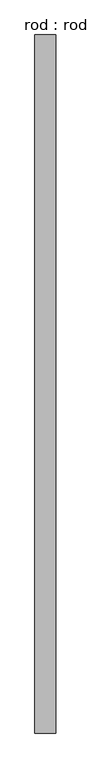
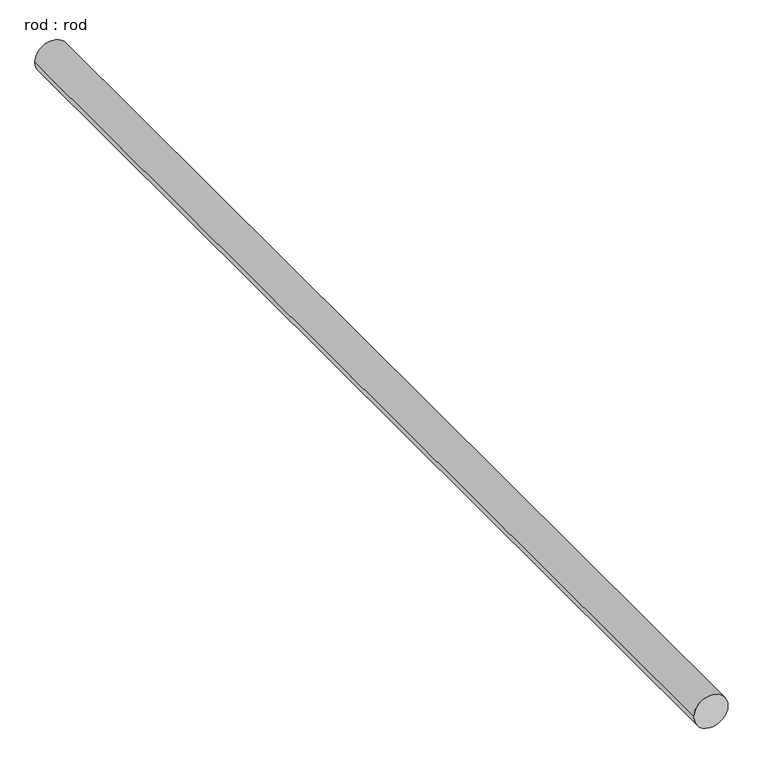
"""IFC4 building model written with IfcOpenShell, lengths in millimetres: proxy geometry, rod : rod."""

from ifc_helpers import new_model, si_unit, point, frame, frame_2d, origin, place, context, project, spatial, circle_curve, trimmed, segment, composite_curve, outline, extrude, source, transform, mapped, element, save


def rod_rod_c0b6d43a(model_context):
    return source(origin(), model_context, "Body", "SweptSolid", [
        extrude(outline(composite_curve([segment(trimmed(circle_curve(frame_2d((0.0108462, 0.0)), 200.0), [point((0.0108462, 200.0))], [point((0.0108462, -200.0))], False, "CARTESIAN"), True, "CONTINUOUS"), segment(trimmed(circle_curve(frame_2d((0.0108462, 0.0)), 200.0), [point((0.0108462, -200.0))], [point((0.0108462, 200.0))], False, "CARTESIAN"), True, "CONTINUOUS")], self_intersect=False)), frame((0.0, -2584.8435406, 0.0), z_axis=(0.0, 1.0, 0.0), x_axis=(0.0, 0.0, 1.0)), (0.0, 0.0, 1.0), 13355.1443119),
    ])


if __name__ == "__main__":
    model = new_model("IFC4")
    model_context = context("Model", 3, world=origin())
    ifc_project = project(units=[si_unit("LENGTHUNIT", "METRE", prefix="MILLI")], contexts=[model_context])
    site = spatial("IfcSite", under=ifc_project)
    building = spatial("IfcBuilding", under=site)
    placement = place(None, origin())
    rod_rod_shape = rod_rod_c0b6d43a(model_context)
    element("IfcBuildingElementProxy", 1, Name="rod : rod", ObjectType="rod : rod", at=placement, inside=building, context=model_context, shape_type="MappedRepresentation", body=[
        mapped(rod_rod_shape, transform((0.0, 0.0, 0.0), x_axis=(1.0, 0.0, 0.0), y_axis=(0.0, 1.0, 0.0), z_axis=(0.0, 0.0, 1.0))),
    ])
    save(model, "model.ifc")

# Revit data of these elements
# Type "rod : rod"
#   Default Elevation = 0
